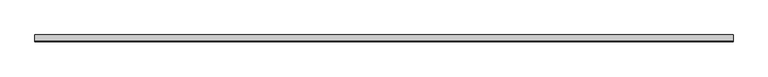
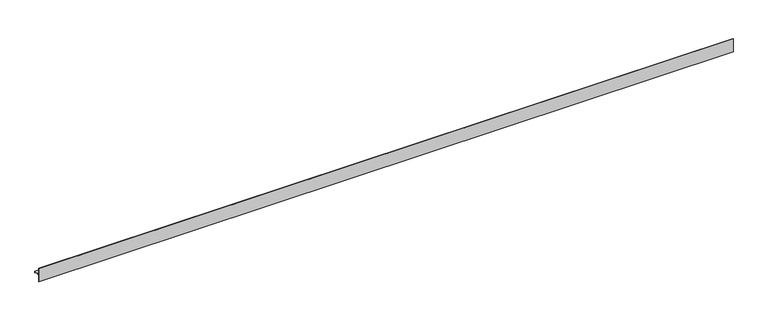
"""IFC4 building model written with IfcOpenShell, lengths in millimetres: proxy geometry, Metal profile004 1127 : Metal profile004 1127."""

from ifc_helpers import new_model, si_unit, frame, origin, place, context, project, spatial, polyline, outline, extrude, source, transform, mapped, element, save


def generic_models_c5715602(model_context):
    return source(origin(), model_context, "Body", "SweptSolid", [
        extrude(outline(polyline([(10464.4562552, 43386.3870313), (10447.4923073, 43386.3870313), (10447.4923073, 43367.3370312), (10446.2223073, 43367.3370312), (10446.2223073, 43406.7070312), (10447.4923073, 43406.7070312), (10447.4923073, 43387.6570312), (10465.7262552, 43387.6570312), (10465.7262552, 43382.9072312), (10464.4562552, 43382.9072312), (10464.4562552, 43386.3870313)])), frame((3694.2883192, 0.0, 0.0), z_axis=(1.0, 0.0, 0.0), x_axis=(0.0, 1.0, 0.0)), (0.0, 0.0, 1.0), 2000.0),
    ])


if __name__ == "__main__":
    model = new_model("IFC4")
    model_context = context("Model", 3, world=origin())
    ifc_project = project(units=[si_unit("LENGTHUNIT", "METRE", prefix="MILLI")], contexts=[model_context])
    site = spatial("IfcSite", under=ifc_project)
    building = spatial("IfcBuilding", under=site)
    placement = place(None, origin())
    generic_models_shape = generic_models_c5715602(model_context)
    element("IfcBuildingElementProxy", 1, Name="Metal profile004 1127 : Metal profile004 1127", ObjectType="Metal profile004 1127 : Metal profile004 1127", at=placement, inside=building, context=model_context, shape_type="MappedRepresentation", body=[
        mapped(generic_models_shape, transform((0.0, 0.0, 0.0), x_axis=(1.0, 0.0, 0.0), y_axis=(0.0, 1.0, 0.0), z_axis=(0.0, 0.0, 1.0))),
    ])
    save(model, "model.ifc")

# Revit data of these elements
# Type "Metal profile004 1127 : Metal profile004 1127"
#   NameOverride = "Metal profile004"
# Element 1 (IfcBuildingElementProxy, "Metal profile004 1127 : Metal profile004 1127")
#   Materials on its faces: "16 GA. COPPER VENTED T REVEAL BEAD"
# Materials
#   "16 GA. COPPER VENTED T REVEAL BEAD": class "Unassigned", colour RGB 255 227 10, transparency 0
